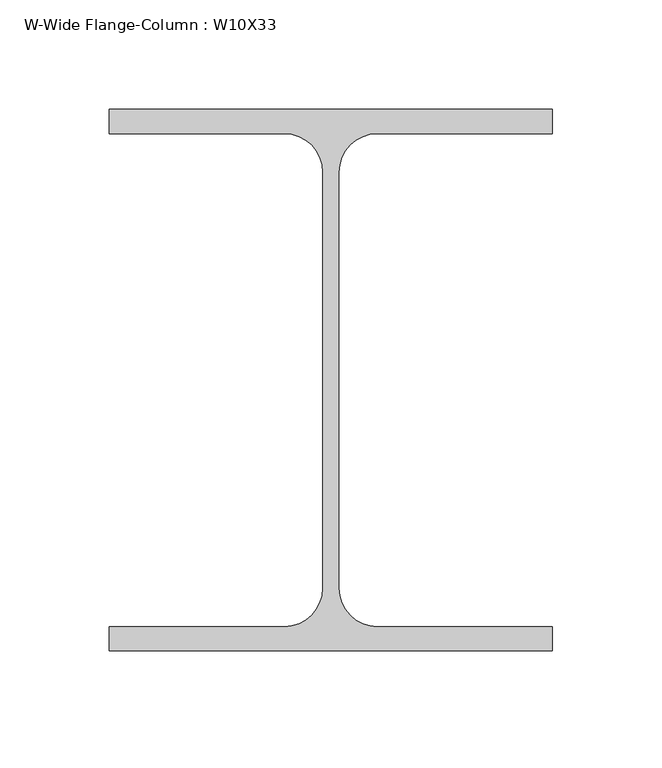
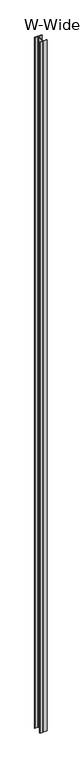
"""IFC4 building model written with IfcOpenShell, lengths in millimetres: column geometry, W-Wide Flange-Column : W10X33."""

from ifc_helpers import new_model, si_unit, point, frame, frame_2d, origin, place, context, project, spatial, polyline, circle_curve, trimmed, segment, composite_curve, outline, extrude, source, transform, mapped, element, save


def w_wide_flange_column_w10x33_7ea207c2(model_context):
    return source(origin(), model_context, "Body", "SweptSolid", [
        extrude(outline(composite_curve([segment(polyline([(101.092, 123.571), (101.092, 112.522), (21.209, 112.522)]), True, "CONTINUOUS"), segment(trimmed(circle_curve(frame_2d((21.209, 94.996)), 17.526), [point((21.209, 112.522))], [point((3.683, 94.996))], True, "CARTESIAN"), True, "CONTINUOUS"), segment(polyline([(3.683, 94.996), (3.683, -94.996)]), True, "CONTINUOUS"), segment(trimmed(circle_curve(frame_2d((21.209, -94.996)), 17.526), [point((3.683, -94.996))], [point((21.209, -112.522))], True, "CARTESIAN"), True, "CONTINUOUS"), segment(polyline([(21.209, -112.522), (101.092, -112.522), (101.092, -123.571), (-101.092, -123.571), (-101.092, -112.522), (-21.209, -112.522)]), True, "CONTINUOUS"), segment(trimmed(circle_curve(frame_2d((-21.209, -94.996)), 17.526), [point((-21.209, -112.522))], [point((-3.683, -94.996))], True, "CARTESIAN"), True, "CONTINUOUS"), segment(polyline([(-3.683, -94.996), (-3.683, 94.996)]), True, "CONTINUOUS"), segment(trimmed(circle_curve(frame_2d((-21.209, 94.996)), 17.526), [point((-3.683, 94.996))], [point((-21.209, 112.522))], True, "CARTESIAN"), True, "CONTINUOUS"), segment(polyline([(-21.209, 112.522), (-101.092, 112.522), (-101.092, 123.571), (101.092, 123.571)]), True, "CONTINUOUS")], self_intersect=False)), frame((0.0, 0.0, 9163.05), z_axis=(0.0, 0.0, 1.0), x_axis=(1.0, 0.0, 0.0)), (0.0, 0.0, 1.0), 20402.55),
    ])


if __name__ == "__main__":
    model = new_model("IFC4")
    model_context = context("Model", 3, world=origin())
    ifc_project = project(units=[si_unit("LENGTHUNIT", "METRE", prefix="MILLI")], contexts=[model_context])
    site = spatial("IfcSite", under=ifc_project)
    building = spatial("IfcBuilding", under=site)
    placement = place(None, origin())
    w_wide_flange_column_w10x33_shape = w_wide_flange_column_w10x33_7ea207c2(model_context)
    element("IfcColumn", 1, ObjectType="W-Wide Flange-Column : W10X33", at=placement, inside=building, context=model_context, shape_type="MappedRepresentation", body=[
        mapped(w_wide_flange_column_w10x33_shape, transform((0.0, 0.0, 0.0), x_axis=(1.0, 0.0, 0.0), y_axis=(0.0, 1.0, 0.0), z_axis=(0.0, 0.0, 1.0))),
    ])
    save(model, "model.ifc")

# Revit data of these elements
# Type "W-Wide Flange-Column : W10X33"
#   Assembly Code = "B10"
#   W = 33
#   bf = 0' - 7.96"
#   d = 0' - 9.73"
#   k = 0' - 1 1/8"
#   kr = 0' - 0.69"
#   tf = 0' - 0.435"
#   tw = 0' - 0.29"
#   A = 0.0674306 SF
#   Structural Material [instance default] = Steel ASTM A992
# Element 1 (IfcColumn, "W-Wide Flange-Column : W10X33")
#   Materials on its faces: "Steel ASTM A992"
# Materials
#   "Steel ASTM A992": class "Metal", colour RGB 199 199 199, transparency 0, Description = "Structural steel 50ksi", Cost = 0
